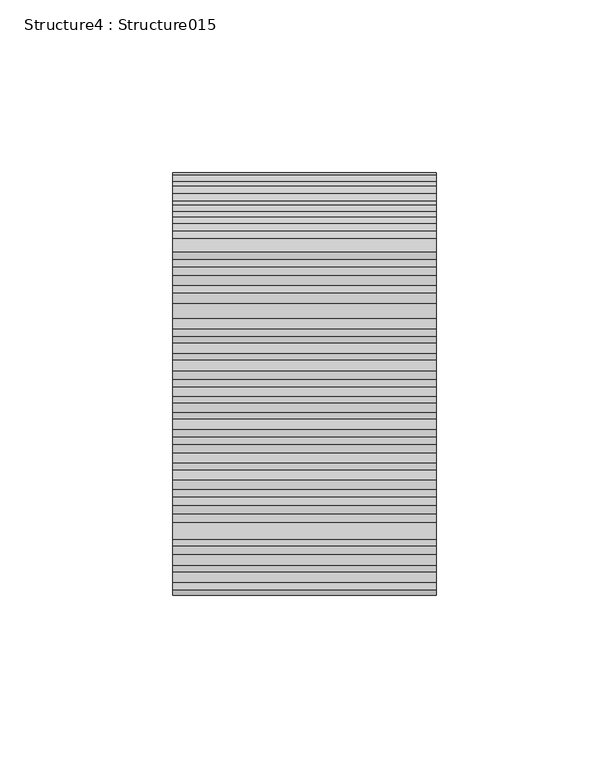
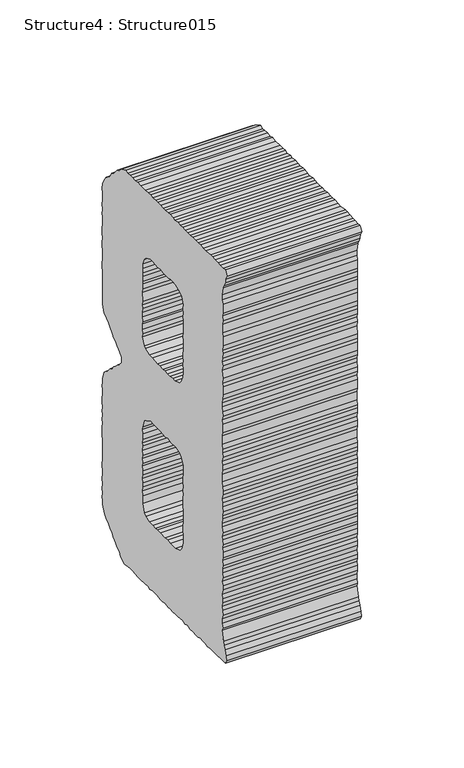
"""IFC4 building model written with IfcOpenShell, lengths in millimetres: proxy geometry, Structure4 : Structure015."""

from ifc_helpers import new_model, si_unit, frame, origin, place, context, project, spatial, polyline, outline, extrude, source, transform, mapped, element, save


def structure4_structure015_850b81e3(model_context):
    return source(origin(), model_context, "Body", "SweptSolid", [
        extrude(outline(polyline([(2.43115, 0.0), (5.2431083, -0.4799365), (7.6490828, -0.4854213), (10.0019016, -1.3619332), (12.0096035, -0.8876659), (15.3101936, -0.9773732), (17.6742477, -1.415143), (20.0159853, -2.3008543), (22.4634745, -1.858976), (26.6992916, -3.5726126), (28.4394267, -6.1502044), (29.7729262, -8.2538859), (31.3514058, -10.155295), (32.7906624, -11.3916274), (34.6057588, -13.0966058), (36.1505457, -15.4388845), (39.3069637, -19.2410509), (40.6485802, -21.35451), (42.309302, -22.3761602), (43.6096498, -24.9213631), (46.5707194, -28.4882162), (48.8331791, -30.2347095), (50.2157692, -31.9001535), (51.5085412, -34.4362307), (53.7710009, -36.182724), (54.7216257, -37.8092854), (56.9274189, -39.9848903), (57.8785849, -41.6121036), (59.4565233, -43.5128609), (61.0010639, -45.8707588), (62.1807298, -47.2917639), (64.2478411, -48.8029439), (65.3452648, -51.1037079), (67.5996075, -52.8404235), (69.1443944, -55.1827023), (70.9594908, -56.8876807), (72.5374292, -58.788438), (73.4470804, -60.8630144), (74.8296706, -62.5284585), (76.8555133, -64.4713823), (78.4676856, -65.9319218), (80.0119313, -68.2735487), (81.1506235, -70.1425688), (89.2524391, -79.9018753), (88.1910454, -81.9908727), (85.8416213, -83.5283787), (82.913728, -84.3690707), (80.6540113, -85.0371364), (78.7856431, -86.1752876), (73.5034679, -88.5410023), (72.4800835, -90.2009615), (70.1790982, -91.3007711), (68.0365093, -93.0794693), (66.5320691, -95.1387833), (64.2006503, -96.6767569), (62.3212008, -97.8241072), (60.858681, -99.4511363), (58.9592274, -101.0279924), (56.8542422, -102.3625742), (54.8720053, -104.8185374), (52.9627741, -106.4035105), (50.8984057, -107.3068895), (49.3835361, -109.3748617), (47.0521173, -110.9128352), (45.1533155, -112.4891503), (43.9165774, -113.9133287), (41.3407197, -115.6542264), (40.1144111, -117.0697466), (37.7241241, -119.0540746), (35.6260629, -120.3983232), (34.1663967, -122.0075684), (31.8173782, -123.5601525), (30.1927971, -124.4959206), (28.6811866, -126.561187), (25.9102266, -128.0511523), (24.2447827, -129.4337424), (22.3005551, -131.4606674), (20.8723798, -132.6462857), (19.1650154, -134.4611607), (16.8225153, -136.0083336), (14.9237135, -137.5846486), (13.0553452, -138.7227998), (11.306466, -140.985038), (9.6514515, -142.3589699), (7.5429609, -143.7118767), (5.1974478, -145.2461358), (1.6286392, -148.2088289), (-0.0704975, -150.0322885), (-2.4575254, -152.0139108), (-4.3187234, -153.1461095), (-6.0682545, -155.4088889), (-8.1728339, -156.7585488), (-9.5944909, -157.9387558), (-11.9400039, -159.4730149), (-15.9787873, -162.8258636), (-17.2151195, -164.2651201), (-21.2539028, -167.6179688), (-23.3673619, -168.9595852), (-24.8711503, -171.0183581), (-26.9659522, -172.3599011), (-29.3153763, -173.8974069), (-31.2174373, -175.4764277), (-32.6871273, -177.1094092), (-34.6278495, -179.1180091), (-38.4397934, -182.2825441), (-40.0574505, -183.2279791), (-42.2426117, -185.4395033), (-45.9711204, -187.7243902), (-47.9637868, -190.1890114), (-50.020985, -191.0864381), (-51.4835048, -192.7134671), (-53.6686659, -194.9249913), (-55.2961006, -195.8785432), (-57.2361709, -197.8866021), (-61.2821244, -201.2454032), (-63.1533461, -202.4013381), (-67.1882184, -205.75094), (-68.6700472, -207.3785836), (-71.0008142, -208.9160161), (-72.2375522, -210.3401944), (-76.2730763, -213.6903374), (-78.3478741, -214.6023745), (-80.7277317, -216.5780444), (-83.6946918, -220.2643874), (-84.5228386, -222.1608528), (-85.6431005, -224.6962046), (-87.350465, -226.5110797), (-88.4602975, -229.0377734), (-91.6021962, -229.6432256), (-92.7376294, -227.7714999), (-94.7138403, -225.3909905), (-96.1493213, -224.1658376), (-98.1260734, -221.7846764), (-99.9373695, -220.0776441), (-101.1251524, -218.6468614), (-103.8005146, -214.4453403), (-105.38657, -212.5348054), (-107.4455643, -211.0334029), (-108.798262, -208.9291431), (-110.1808521, -207.2636991), (-112.1880377, -205.3207017), (-113.4883857, -202.7754989), (-115.1186739, -201.3156846), (-116.6448037, -198.9733325), (-118.4785572, -197.2684275), (-119.8611472, -195.6029835), (-121.4776362, -194.1306125), (-122.9733325, -191.3500965), (-124.4006965, -190.1347211), (-126.415458, -188.1825981), (-127.6026997, -186.7524673), (-129.1507458, -184.4128942), (-130.5333359, -182.7474502), (-132.3451732, -181.039766), (-134.0885676, -178.4648798), (-135.5015912, -177.2375996), (-136.9972875, -174.4570836), (-138.6661261, -173.4256558), (-140.0487163, -171.7602117), (-141.7996865, -169.1761997), (-144.557832, -165.8537855), (-146.7679418, -163.6663491), (-147.6694761, -161.6015504), (-149.6910021, -159.6704579), (-151.2770575, -157.759923), (-152.4119495, -155.8888492), (-154.2761365, -154.6221081), (-155.4176823, -150.3397219), (-155.1348285, -147.2916877), (-155.5662774, -144.8355404), (-155.0776457, -142.0141613), (-154.6401956, -139.6470695), (-155.1130238, -137.6238589), (-154.0004732, -135.0938077), (-154.1875939, -132.4359292), (-154.3863369, -129.7865979), (-153.5167861, -127.4439624), (-151.8360797, -123.6472808), (-149.8616647, -121.1978113), (-147.790778, -120.2890209), (-145.6547075, -118.5157341), (-144.4179695, -117.0915557), (-142.7103588, -115.2610614), (-140.1347473, -113.5357829), (-138.4382178, -111.7144878), (-136.5594203, -110.5676786), (-134.2280014, -109.0297049), (-130.81433, -105.3854179), (-129.1488859, -104.0028278), (-126.7994619, -102.4653218), (-125.3362901, -100.8377516), (-123.6708461, -99.4551616), (-121.1365031, -98.1616269), (-119.2370495, -96.5847707), (-117.2858979, -94.5675126), (-115.5789391, -92.7375594), (-113.6768781, -91.1585387), (-111.8078581, -90.0198464), (-109.6724394, -88.2471007), (-107.8109953, -87.0992827), (-98.0510369, -78.996926), (-96.5731191, -77.3725291), (-92.2528094, -75.7899047), (-89.4911347, -76.7079678), (-87.1072305, -77.1457748), (-84.7427708, -77.5986227), (-81.8823737, -77.6408628), (-79.2319602, -77.4434235), (-77.2878433, -77.8488414), (-74.9133598, -78.2779531), (-71.9056476, -79.0082809), (-69.0114469, -78.6084585), (-66.3949724, -76.436358), (-65.9576331, -74.0704592), (-66.1865635, -71.8436726), (-65.9108797, -68.8015908), (-65.9031932, -66.3783737), (-65.417415, -63.5747785), (-65.6650024, -61.3480654), (-64.9419556, -58.3474985), (-65.1715378, -56.121253), (-65.1213897, -53.2664027), (-62.3355731, -49.3472678), (-60.4335122, -47.7682472), (-59.4094758, -46.1077469), (-57.2973205, -44.7672126), (-55.3978669, -43.1903564), (-53.6915599, -41.3609444), (-51.5515784, -39.5844108), (-49.4498525, -38.2525346), (-47.7428936, -36.4225815), (-45.6863473, -35.5256959), (-43.9381199, -33.2639989), (-41.8253128, -31.9229236), (-40.60658, -30.4982776), (-36.3168394, -26.9370935), (-34.2602931, -26.040208), (-25.2173556, -18.5330955), (-23.2246892, -16.0684743), (-19.0249022, -13.3923495), (-16.3256443, -10.3411421), (-14.2232666, -9.0087249), (-12.0463331, -6.7886161), (-9.7453479, -5.6888064), (-8.2337374, -3.62354), (-6.1700208, -2.720702), (-4.5045767, -1.3381119), (0.0, 0.0), (2.43115, 0.0)]), holes=[polyline([(-76.2863159, -111.9905152), (-78.3926047, -113.3261792), (-80.7724623, -115.301849), (-81.5580368, -116.7654884), (-84.1033504, -118.0670292), (-86.0132334, -119.6525435), (-87.7537494, -121.90894), (-89.570309, -122.6054962), (-91.0852893, -124.6746613), (-95.2856176, -127.3501342), (-96.7966869, -129.4160525), (-99.1286468, -130.9533742), (-100.3241162, -131.9458087), (-102.5080844, -134.1574436), (-104.1741802, -135.5405748), (-106.2721307, -136.8836305), (-108.4186306, -138.6655754), (-110.0813318, -142.4627246), (-110.2505633, -144.2085659), (-109.1100749, -148.4764151), (-107.7193678, -150.1516368), (-105.9074198, -151.8581279), (-103.896975, -153.7984197), (-102.9768944, -155.8643379), (-100.5370917, -157.8456768), (-97.3730978, -161.6569689), (-96.6564826, -163.4777964), (-95.078003, -165.3792056), (-93.2655138, -167.0863486), (-89.0601303, -169.238149), (-86.6856468, -169.6672607), (-82.8426176, -168.4951707), (-81.1434807, -166.671711), (-78.8452135, -165.5752588), (-77.334796, -163.5098817), (-75.5136736, -162.8095375), (-69.7918467, -158.0594883), (-68.2879475, -155.9995224), (-66.2341192, -155.1059944), (-62.6587922, -152.1378901), (-59.2456619, -148.4929511), (-56.7107778, -147.2000683), (-55.4330661, -145.327875), (-52.8988338, -144.0355333), (-51.4667475, -142.8466681), (-49.4850516, -140.3900532), (-47.8522428, -137.0317197), (-47.4149036, -134.6658208), (-49.2293482, -130.5291513), (-50.6049036, -128.8721811), (-52.1503423, -126.5304436), (-53.7282807, -124.6296863), (-55.3549529, -123.1503541), (-56.5015779, -121.2890207), (-58.7067192, -119.1128745), (-59.8614612, -117.2417635), (-63.4982832, -113.8384107), (-65.2796869, -111.6925627), (-69.0279297, -109.57416), (-70.3388178, -109.4699582), (-74.8172777, -110.3580748), (-76.2863159, -111.9905152)]), polyline([(-35.5495712, -82.5920473), (-34.6518125, -87.0768165), (-33.2202425, -88.3052161), (-31.642304, -90.2059734), (-30.1122632, -92.5450788), (-28.4777691, -94.0179173), (-26.7044822, -96.1539878), (-24.892645, -97.8616719), (-23.9790828, -99.9330016), (-21.5333027, -101.9082773), (-18.5641161, -105.484908), (-15.0427127, -107.7916244), (-13.1067128, -108.1872648), (-9.0585577, -107.242371), (-6.9599554, -105.8987741), (-4.8167147, -104.1195349), (-3.3062971, -102.0541578), (-1.6473714, -100.676979), (1.1312998, -99.1817131), (2.3979302, -97.3187191), (4.4628397, -96.4159918), (5.9732572, -94.3506147), (9.5420659, -91.3879217), (12.0873794, -90.0863808), (13.9861812, -88.5100657), (15.4492174, -86.8969218), (17.3209803, -85.7416387), (18.8216202, -83.6843786), (20.7308514, -82.0994054), (23.0698461, -80.5705575), (26.8824419, -77.4054814), (29.1834271, -73.8745218), (29.4254182, -71.2733097), (27.8551663, -66.9493352), (24.6906313, -63.1373912), (22.631637, -61.6359888), (21.2900205, -59.5225298), (18.3289509, -55.9556766), (16.3031082, -54.0127528), (15.4091498, -51.9570796), (13.5864774, -50.2429754), (11.3652864, -48.0647384), (8.283424, -45.8060303), (6.3061556, -45.8421338), (1.7874847, -47.1765313), (-1.777413, -50.1359776), (-4.1268371, -51.6734835), (-5.8337959, -53.5034368), (-7.7365087, -55.0829986), (-9.848664, -56.4235327), (-11.3525631, -58.4834987), (-13.2034673, -59.6214656), (-15.5528914, -61.1589715), (-16.5829048, -62.825535), (-19.1217001, -64.1216646), (-20.3955006, -65.9906111), (-22.697027, -67.0897689), (-24.6366917, -69.112906), (-26.2612729, -70.0486741), (-27.7756014, -72.1172981), (-30.1561108, -74.093509), (-32.4537262, -75.18942), (-33.4869989, -76.8586892), (-36.0219937, -80.5839149), (-35.5495712, -82.5920473)])]), frame((-35624.0862846, 278152.3913276, 4000.7739371), z_axis=(1.0, 0.0, 1.354250045437766e-12), x_axis=(1.0299598056967423e-12, -0.6387436987479043, -0.7694195781950487)), (0.0, 0.0, 1.0), 76.2),
    ])


if __name__ == "__main__":
    model = new_model("IFC4")
    model_context = context("Model", 3, world=origin())
    ifc_project = project(units=[si_unit("LENGTHUNIT", "METRE", prefix="MILLI")], contexts=[model_context])
    site = spatial("IfcSite", under=ifc_project)
    building = spatial("IfcBuilding", under=site)
    placement = place(None, origin())
    structure4_structure015_shape = structure4_structure015_850b81e3(model_context)
    element("IfcBuildingElementProxy", 1, Name="Structure4 : Structure015", ObjectType="Structure4 : Structure015", at=placement, inside=building, context=model_context, shape_type="MappedRepresentation", body=[
        mapped(structure4_structure015_shape, transform((0.0, 0.0, 0.0), x_axis=(1.0, 0.0, 0.0), y_axis=(0.0, 1.0, 0.0), z_axis=(0.0, 0.0, 1.0))),
    ])
    save(model, "model.ifc")

# Revit data of these elements
# Type "Structure4 : Structure015"
#   NameOverride = "Structure015"
# Element 1 (IfcBuildingElementProxy, "Structure4 : Structure015")
#   Materials on its faces: "BRUSHED ALUMINUM LETTERING"
# Materials
#   "BRUSHED ALUMINUM LETTERING": class "Unassigned", colour RGB 169 181 186, transparency 0, Cost = 0
